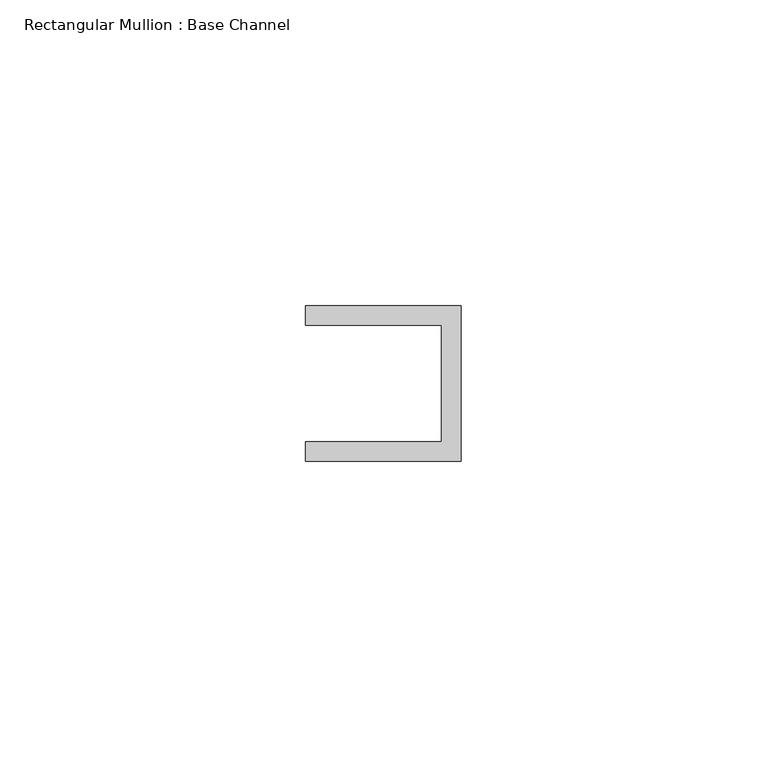
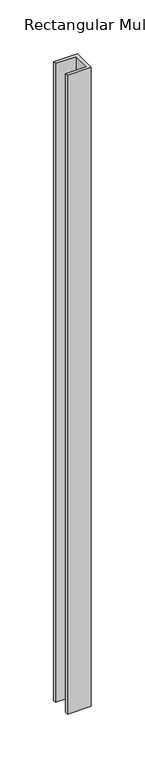
"""IFC4 building model written with IfcOpenShell, lengths in millimetres: member geometry, Rectangular Mullion : Base Channel."""

import ifcopenshell
import ifcopenshell.guid

model = None  # the IFC model being written
_history = None  # IfcOwnerHistory: only IFC2X3 demands one
_inside = {}  # id of a spatial element -> (the spatial element, [elements in it])
_under = {}  # id of a project, library or spatial element -> (it, [spatial elements below it])
_declared = {}  # id of a project -> (the project, [libraries it declares])
_typed = {}  # id of a type object -> (the type object, [elements of that type])
_made_of = {}  # id of a material, layer set ... -> (it, [elements and type objects made of it])


def new_model(schema):
    """Start an empty IFC model of exactly this schema.

    Asked for "IFC4X3", IfcOpenShell would pick the latest addendum, in which some entities
    have other attributes; the version numbers below select the first issue.
    IFC2X3 requires an IfcOwnerHistory on every rooted entity: one is made here for all.
    """
    global model, _history
    if schema == "IFC4X3":
        model = ifcopenshell.file(schema_version=(4, 3, 0, 0))
    else:
        model = ifcopenshell.file(schema=schema)
    _inside.clear()
    _under.clear()
    _declared.clear()
    _typed.clear()
    _made_of.clear()
    _history = None
    if model.schema == "IFC2X3":
        org = make("IfcOrganization", Name="unknown")
        user = make(
            "IfcPersonAndOrganization",
            ThePerson=make("IfcPerson", FamilyName="unknown"),
            TheOrganization=org,
        )
        app = make(
            "IfcApplication",
            ApplicationDeveloper=org,
            Version="unknown",
            ApplicationFullName="unknown",
            ApplicationIdentifier="unknown",
        )
        _history = make(
            "IfcOwnerHistory",
            OwningUser=user,
            OwningApplication=app,
            ChangeAction="ADDED",
            CreationDate=0,
        )
    return model


def make(cls, **values):
    """One entity of the class cls with the attributes given. An attribute that is None is left unset."""
    return model.create_entity(
        cls, **{name: value for name, value in values.items() if value is not None}
    )


def rooted(cls, **values):
    """An entity with a GlobalId (a new one), such as an element, a storey or a relation."""
    return make(cls, GlobalId=ifcopenshell.guid.new(), OwnerHistory=_history, **values)


def si_unit(unit_type, name, prefix=None):
    """IfcSIUnit, for example si_unit("LENGTHUNIT", "METRE", prefix="MILLI")."""
    return make("IfcSIUnit", UnitType=unit_type, Prefix=prefix, Name=name)


def assignment(units):
    """IfcUnitAssignment: the units of a project."""
    return None if units is None else make("IfcUnitAssignment", Units=units)


def point(xyz):
    """IfcCartesianPoint."""
    return None if xyz is None else make("IfcCartesianPoint", Coordinates=xyz)


def direction(xyz):
    """IfcDirection."""
    return None if xyz is None else make("IfcDirection", DirectionRatios=xyz)


def frame(location, z_axis=None, x_axis=None):
    """IfcAxis2Placement3D, a coordinate frame: its origin and axes. An axis left out is left unset."""
    return make(
        "IfcAxis2Placement3D",
        Location=point(location),
        Axis=direction(z_axis),
        RefDirection=direction(x_axis),
    )


def origin():
    """The frame at (0, 0, 0) with its axes left unset."""
    return frame((0.0, 0.0, 0.0))


def place(relative_to, where):
    """IfcLocalPlacement: puts the frame where relative to a parent placement (None: the world)."""
    return make(
        "IfcLocalPlacement", PlacementRelTo=relative_to, RelativePlacement=where
    )


def context(
    kind, dimensions, precision=None, world=None, true_north=None, identifier=None
):
    """IfcGeometricRepresentationContext, for example the 3D "Model" context."""
    return make(
        "IfcGeometricRepresentationContext",
        ContextIdentifier=identifier,
        ContextType=kind,
        CoordinateSpaceDimension=dimensions,
        Precision=precision,
        WorldCoordinateSystem=world,
        TrueNorth=true_north,
    )


def project(units=None, contexts=None):
    """IfcProject with its units and contexts."""
    return rooted(
        "IfcProject",
        Name="project",
        RepresentationContexts=contexts,
        UnitsInContext=assignment(units),
    )


def spatial(cls, under=None, at=None, **own):
    """A site, building, storey or space (cls), placed at a placement, below another one or the project."""
    s = rooted(cls, ObjectPlacement=at, **own)
    if under is not None:
        _under.setdefault(under.id(), (under, []))[1].append(s)
    return s


def polyline(points):
    """IfcPolyline through the points."""
    return make("IfcPolyline", Points=[point(p) for p in points])


def outline(outer, holes=None, kind="AREA"):
    """IfcArbitraryClosedProfileDef: a profile drawn as a closed curve; with holes, ...WithVoids."""
    if holes is None:
        return make("IfcArbitraryClosedProfileDef", ProfileType=kind, OuterCurve=outer)
    return make(
        "IfcArbitraryProfileDefWithVoids",
        ProfileType=kind,
        OuterCurve=outer,
        InnerCurves=holes,
    )


def extrude(swept, where, along, depth):
    """IfcExtrudedAreaSolid: the profile swept, set in the frame where, extruded along a direction by depth."""
    return make(
        "IfcExtrudedAreaSolid",
        SweptArea=swept,
        Position=where,
        ExtrudedDirection=direction(along),
        Depth=depth,
    )


def shape(context_of_items, identifier, shape_type, items):
    """IfcShapeRepresentation: the items that make up one representation, for example the "Body"."""
    return make(
        "IfcShapeRepresentation",
        ContextOfItems=context_of_items,
        RepresentationIdentifier=identifier,
        RepresentationType=shape_type,
        Items=items,
    )


def source(mapping_origin, context_of_items, identifier, shape_type, items):
    """IfcRepresentationMap: a shape defined once, which mapped items show again and again."""
    return make(
        "IfcRepresentationMap",
        MappingOrigin=mapping_origin,
        MappedRepresentation=shape(context_of_items, identifier, shape_type, items),
    )


def transform(
    local_origin,
    x_axis=None,
    y_axis=None,
    z_axis=None,
    scale=None,
    scale2=None,
    scale3=None,
    uniform=True,
):
    """IfcCartesianTransformationOperator3D, or its non-uniform kind. x_axis, y_axis, z_axis: its Axis1, 2, 3."""
    if uniform:
        return make(
            "IfcCartesianTransformationOperator3D",
            Axis1=direction(x_axis),
            Axis2=direction(y_axis),
            LocalOrigin=point(local_origin),
            Scale=scale,
            Axis3=direction(z_axis),
        )
    return make(
        "IfcCartesianTransformationOperator3DnonUniform",
        Axis1=direction(x_axis),
        Axis2=direction(y_axis),
        LocalOrigin=point(local_origin),
        Scale=scale,
        Axis3=direction(z_axis),
        Scale2=scale2,
        Scale3=scale3,
    )


def mapped(mapping_source, mapping_target):
    """IfcMappedItem: shows the shape of a source again, moved by a transform."""
    return make(
        "IfcMappedItem", MappingSource=mapping_source, MappingTarget=mapping_target
    )


def made_of(thing, what):
    """Note that an element or type object is made of a material, layer set ...; save() writes the relation."""
    if what is not None:
        _made_of.setdefault(what.id(), (what, []))[1].append(thing)
    return thing


def element(
    cls,
    number,
    at=None,
    inside=None,
    cuts=None,
    type_object=None,
    material=None,
    context=None,
    identifier="Body",
    shape_type=None,
    held_by="IfcProductDefinitionShape",
    body=None,
    shapes=None,
    **own,
):
    """One element of the class cls, such as IfcWall. Its Tag is "e" and its number.

    at: its placement. inside: the storey or other place that contains it. cuts: it is an
    opening in that element (IfcRelVoidsElement). A single representation is given by context,
    identifier, shape_type and body (its items); several are given by shapes. held_by: the class
    of the entity that holds the representations. save() writes the other relations.
    """
    e = rooted(cls, Tag="e%d" % number, ObjectPlacement=at, **own)
    if body is not None:
        shapes = [shape(context, identifier, shape_type, body)]
    if shapes is not None:
        e.Representation = make(held_by, Representations=shapes)
    if inside is not None:
        _inside.setdefault(inside.id(), (inside, []))[1].append(e)
    if cuts is not None:
        rooted(
            "IfcRelVoidsElement", RelatingBuildingElement=cuts, RelatedOpeningElement=e
        )
    if type_object is not None:
        _typed.setdefault(type_object.id(), (type_object, []))[1].append(e)
    return made_of(e, material)


def aggregate(whole, parts):
    """IfcRelAggregates: a whole, such as a stair, and the parts it consists of."""
    return rooted("IfcRelAggregates", RelatingObject=whole, RelatedObjects=parts)


def save(model, path):
    """Write the relations noted so far, then the file.

    IfcRelAggregates (storeys below a building ...), IfcRelContainedInSpatialStructure (elements
    in a storey), IfcRelDefinesByType, IfcRelAssociatesMaterial and IfcRelDeclares: one each for
    every whole, place, type object, material and project.
    """
    for whole, parts in _under.values():
        aggregate(whole, parts)
    for where, things in _inside.values():
        rooted(
            "IfcRelContainedInSpatialStructure",
            RelatedElements=things,
            RelatingStructure=where,
        )
    for kind, things in _typed.values():
        rooted("IfcRelDefinesByType", RelatedObjects=things, RelatingType=kind)
    for what, things in _made_of.values():
        rooted("IfcRelAssociatesMaterial", RelatedObjects=things, RelatingMaterial=what)
    for by, libraries in _declared.values():
        rooted("IfcRelDeclares", RelatingContext=by, RelatedDefinitions=libraries)
    model.write(path)


def rectangular_mullion_base_channel_6cbbcb1d(model_context):
    return source(origin(), model_context, "Body", "SweptSolid", [
        extrude(outline(polyline([(0.0, -12.7), (-25.4, -12.7), (-25.4, -9.525), (-3.175, -9.525), (-3.175, 9.525), (-25.4, 9.525), (-25.4, 12.7), (0.0, 12.7), (0.0, -12.7)])), frame((0.0, 0.0, -723.9), z_axis=(0.0, 0.0, 1.0), x_axis=(1.0, 0.0, 0.0)), (0.0, 0.0, 1.0), 723.9),
    ])


if __name__ == "__main__":
    model = new_model("IFC4")
    model_context = context("Model", 3, world=origin())
    ifc_project = project(units=[si_unit("LENGTHUNIT", "METRE", prefix="MILLI")], contexts=[model_context])
    site = spatial("IfcSite", under=ifc_project)
    building = spatial("IfcBuilding", under=site)
    placement = place(None, origin())
    rectangular_mullion_base_channel_shape = rectangular_mullion_base_channel_6cbbcb1d(model_context)
    element("IfcMember", 1, ObjectType="Rectangular Mullion : Base Channel", at=placement, inside=building, context=model_context, shape_type="MappedRepresentation", body=[
        mapped(rectangular_mullion_base_channel_shape, transform((0.0, 0.0, 0.0), x_axis=(1.0, 0.0, 0.0), y_axis=(0.0, 1.0, 0.0), z_axis=(0.0, 0.0, 1.0))),
    ])
    save(model, "model.ifc")

# Revit data of these elements
# Type "Rectangular Mullion : Base Channel"
#   built-in parameter 1007322 = 0.0833333 (stored number, unit not read)
#   built-in parameter 1007321 = 0.0416667 (stored number, unit not read)
#   built-in parameter 1007320 = -0.03125 (stored number, unit not read)
# Element 1 (IfcMember, "Rectangular Mullion : Base Channel")
#   Materials on its faces: "ALUM"
# Materials
#   "ALUM": class "Generic", colour RGB 157 157 157, transparency 0, Cost = 0
